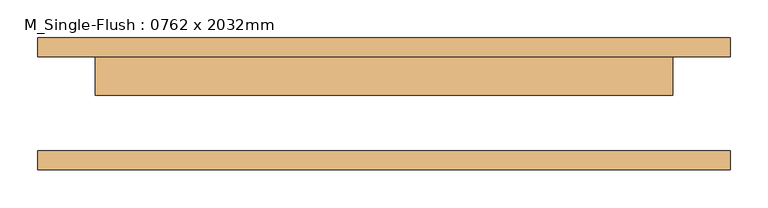
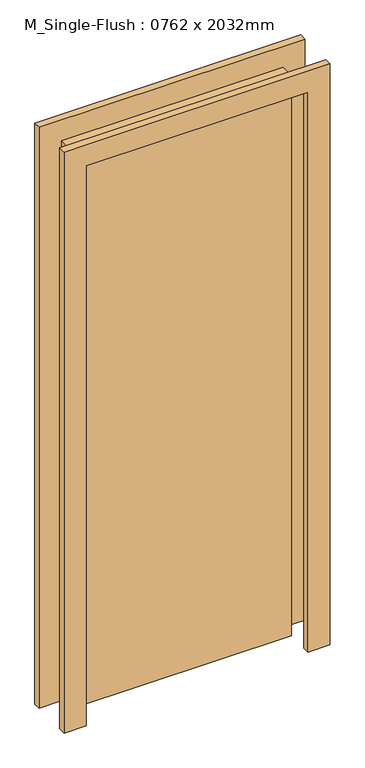
"""IFC4 building model written with IfcOpenShell, lengths in millimetres: door geometry, M_Single-Flush : 0762 x 2032mm."""

import ifcopenshell
import ifcopenshell.guid

model = None  # the IFC model being written
_history = None  # IfcOwnerHistory: only IFC2X3 demands one
_inside = {}  # id of a spatial element -> (the spatial element, [elements in it])
_under = {}  # id of a project, library or spatial element -> (it, [spatial elements below it])
_declared = {}  # id of a project -> (the project, [libraries it declares])
_typed = {}  # id of a type object -> (the type object, [elements of that type])
_made_of = {}  # id of a material, layer set ... -> (it, [elements and type objects made of it])


def new_model(schema):
    """Start an empty IFC model of exactly this schema.

    Asked for "IFC4X3", IfcOpenShell would pick the latest addendum, in which some entities
    have other attributes; the version numbers below select the first issue.
    IFC2X3 requires an IfcOwnerHistory on every rooted entity: one is made here for all.
    """
    global model, _history
    if schema == "IFC4X3":
        model = ifcopenshell.file(schema_version=(4, 3, 0, 0))
    else:
        model = ifcopenshell.file(schema=schema)
    _inside.clear()
    _under.clear()
    _declared.clear()
    _typed.clear()
    _made_of.clear()
    _history = None
    if model.schema == "IFC2X3":
        org = make("IfcOrganization", Name="unknown")
        user = make(
            "IfcPersonAndOrganization",
            ThePerson=make("IfcPerson", FamilyName="unknown"),
            TheOrganization=org,
        )
        app = make(
            "IfcApplication",
            ApplicationDeveloper=org,
            Version="unknown",
            ApplicationFullName="unknown",
            ApplicationIdentifier="unknown",
        )
        _history = make(
            "IfcOwnerHistory",
            OwningUser=user,
            OwningApplication=app,
            ChangeAction="ADDED",
            CreationDate=0,
        )
    return model


def make(cls, **values):
    """One entity of the class cls with the attributes given. An attribute that is None is left unset."""
    return model.create_entity(
        cls, **{name: value for name, value in values.items() if value is not None}
    )


def rooted(cls, **values):
    """An entity with a GlobalId (a new one), such as an element, a storey or a relation."""
    return make(cls, GlobalId=ifcopenshell.guid.new(), OwnerHistory=_history, **values)


def si_unit(unit_type, name, prefix=None):
    """IfcSIUnit, for example si_unit("LENGTHUNIT", "METRE", prefix="MILLI")."""
    return make("IfcSIUnit", UnitType=unit_type, Prefix=prefix, Name=name)


def assignment(units):
    """IfcUnitAssignment: the units of a project."""
    return None if units is None else make("IfcUnitAssignment", Units=units)


def point(xyz):
    """IfcCartesianPoint."""
    return None if xyz is None else make("IfcCartesianPoint", Coordinates=xyz)


def direction(xyz):
    """IfcDirection."""
    return None if xyz is None else make("IfcDirection", DirectionRatios=xyz)


def frame(location, z_axis=None, x_axis=None):
    """IfcAxis2Placement3D, a coordinate frame: its origin and axes. An axis left out is left unset."""
    return make(
        "IfcAxis2Placement3D",
        Location=point(location),
        Axis=direction(z_axis),
        RefDirection=direction(x_axis),
    )


def origin():
    """The frame at (0, 0, 0) with its axes left unset."""
    return frame((0.0, 0.0, 0.0))


def origin_with_axes():
    """The frame at (0, 0, 0) with the z axis (0, 0, 1) and the x axis (1, 0, 0) written out."""
    return frame((0.0, 0.0, 0.0), z_axis=(0.0, 0.0, 1.0), x_axis=(1.0, 0.0, 0.0))


def place(relative_to, where):
    """IfcLocalPlacement: puts the frame where relative to a parent placement (None: the world)."""
    return make(
        "IfcLocalPlacement", PlacementRelTo=relative_to, RelativePlacement=where
    )


def context(
    kind, dimensions, precision=None, world=None, true_north=None, identifier=None
):
    """IfcGeometricRepresentationContext, for example the 3D "Model" context."""
    return make(
        "IfcGeometricRepresentationContext",
        ContextIdentifier=identifier,
        ContextType=kind,
        CoordinateSpaceDimension=dimensions,
        Precision=precision,
        WorldCoordinateSystem=world,
        TrueNorth=true_north,
    )


def project(units=None, contexts=None):
    """IfcProject with its units and contexts."""
    return rooted(
        "IfcProject",
        Name="project",
        RepresentationContexts=contexts,
        UnitsInContext=assignment(units),
    )


def spatial(cls, under=None, at=None, **own):
    """A site, building, storey or space (cls), placed at a placement, below another one or the project."""
    s = rooted(cls, ObjectPlacement=at, **own)
    if under is not None:
        _under.setdefault(under.id(), (under, []))[1].append(s)
    return s


def polyline(points):
    """IfcPolyline through the points."""
    return make("IfcPolyline", Points=[point(p) for p in points])


def outline(outer, holes=None, kind="AREA"):
    """IfcArbitraryClosedProfileDef: a profile drawn as a closed curve; with holes, ...WithVoids."""
    if holes is None:
        return make("IfcArbitraryClosedProfileDef", ProfileType=kind, OuterCurve=outer)
    return make(
        "IfcArbitraryProfileDefWithVoids",
        ProfileType=kind,
        OuterCurve=outer,
        InnerCurves=holes,
    )


def extrude(swept, where, along, depth):
    """IfcExtrudedAreaSolid: the profile swept, set in the frame where, extruded along a direction by depth."""
    return make(
        "IfcExtrudedAreaSolid",
        SweptArea=swept,
        Position=where,
        ExtrudedDirection=direction(along),
        Depth=depth,
    )


def shape(context_of_items, identifier, shape_type, items):
    """IfcShapeRepresentation: the items that make up one representation, for example the "Body"."""
    return make(
        "IfcShapeRepresentation",
        ContextOfItems=context_of_items,
        RepresentationIdentifier=identifier,
        RepresentationType=shape_type,
        Items=items,
    )


def source(mapping_origin, context_of_items, identifier, shape_type, items):
    """IfcRepresentationMap: a shape defined once, which mapped items show again and again."""
    return make(
        "IfcRepresentationMap",
        MappingOrigin=mapping_origin,
        MappedRepresentation=shape(context_of_items, identifier, shape_type, items),
    )


def transform(
    local_origin,
    x_axis=None,
    y_axis=None,
    z_axis=None,
    scale=None,
    scale2=None,
    scale3=None,
    uniform=True,
):
    """IfcCartesianTransformationOperator3D, or its non-uniform kind. x_axis, y_axis, z_axis: its Axis1, 2, 3."""
    if uniform:
        return make(
            "IfcCartesianTransformationOperator3D",
            Axis1=direction(x_axis),
            Axis2=direction(y_axis),
            LocalOrigin=point(local_origin),
            Scale=scale,
            Axis3=direction(z_axis),
        )
    return make(
        "IfcCartesianTransformationOperator3DnonUniform",
        Axis1=direction(x_axis),
        Axis2=direction(y_axis),
        LocalOrigin=point(local_origin),
        Scale=scale,
        Axis3=direction(z_axis),
        Scale2=scale2,
        Scale3=scale3,
    )


def mapped(mapping_source, mapping_target):
    """IfcMappedItem: shows the shape of a source again, moved by a transform."""
    return make(
        "IfcMappedItem", MappingSource=mapping_source, MappingTarget=mapping_target
    )


def made_of(thing, what):
    """Note that an element or type object is made of a material, layer set ...; save() writes the relation."""
    if what is not None:
        _made_of.setdefault(what.id(), (what, []))[1].append(thing)
    return thing


def element(
    cls,
    number,
    at=None,
    inside=None,
    cuts=None,
    type_object=None,
    material=None,
    context=None,
    identifier="Body",
    shape_type=None,
    held_by="IfcProductDefinitionShape",
    body=None,
    shapes=None,
    **own,
):
    """One element of the class cls, such as IfcWall. Its Tag is "e" and its number.

    at: its placement. inside: the storey or other place that contains it. cuts: it is an
    opening in that element (IfcRelVoidsElement). A single representation is given by context,
    identifier, shape_type and body (its items); several are given by shapes. held_by: the class
    of the entity that holds the representations. save() writes the other relations.
    """
    e = rooted(cls, Tag="e%d" % number, ObjectPlacement=at, **own)
    if body is not None:
        shapes = [shape(context, identifier, shape_type, body)]
    if shapes is not None:
        e.Representation = make(held_by, Representations=shapes)
    if inside is not None:
        _inside.setdefault(inside.id(), (inside, []))[1].append(e)
    if cuts is not None:
        rooted(
            "IfcRelVoidsElement", RelatingBuildingElement=cuts, RelatedOpeningElement=e
        )
    if type_object is not None:
        _typed.setdefault(type_object.id(), (type_object, []))[1].append(e)
    return made_of(e, material)


def aggregate(whole, parts):
    """IfcRelAggregates: a whole, such as a stair, and the parts it consists of."""
    return rooted("IfcRelAggregates", RelatingObject=whole, RelatedObjects=parts)


def save(model, path):
    """Write the relations noted so far, then the file.

    IfcRelAggregates (storeys below a building ...), IfcRelContainedInSpatialStructure (elements
    in a storey), IfcRelDefinesByType, IfcRelAssociatesMaterial and IfcRelDeclares: one each for
    every whole, place, type object, material and project.
    """
    for whole, parts in _under.values():
        aggregate(whole, parts)
    for where, things in _inside.values():
        rooted(
            "IfcRelContainedInSpatialStructure",
            RelatedElements=things,
            RelatingStructure=where,
        )
    for kind, things in _typed.values():
        rooted("IfcRelDefinesByType", RelatedObjects=things, RelatingType=kind)
    for what, things in _made_of.values():
        rooted("IfcRelAssociatesMaterial", RelatedObjects=things, RelatingMaterial=what)
    for by, libraries in _declared.values():
        rooted("IfcRelDeclares", RelatingContext=by, RelatedDefinitions=libraries)
    model.write(path)


def m_single_flush_0762_x_2032mm_e53dc8c7(model_context):
    return source(origin(), model_context, "Body", "SweptSolid", [
        extrude(outline(polyline([(2108.0, -457.0), (0.0, -457.0), (0.0, -381.0), (2032.0, -381.0), (2032.0, 381.0), (0.0, 381.0), (0.0, 457.0), (2108.0, 457.0), (2108.0, -457.0)])), frame((0.0, 62.0, 0.0), z_axis=(0.0, 1.0, 0.0), x_axis=(0.0, 0.0, 1.0)), (0.0, 0.0, 1.0), 25.0),
        extrude(outline(polyline([(2108.0, 457.0), (2108.0, -457.0), (0.0, -457.0), (0.0, -381.0), (2032.0, -381.0), (2032.0, 381.0), (0.0, 381.0), (0.0, 457.0), (2108.0, 457.0)])), frame((0.0, -87.0, 0.0), z_axis=(0.0, 1.0, 0.0), x_axis=(0.0, 0.0, 1.0)), (0.0, 0.0, 1.0), 25.0),
        extrude(outline(polyline([(381.0, 11.0), (-381.0, 11.0), (-381.0, 62.0), (381.0, 62.0), (381.0, 11.0)])), origin_with_axes(), (0.0, 0.0, 1.0), 2032.0),
    ])


if __name__ == "__main__":
    model = new_model("IFC4")
    model_context = context("Model", 3, world=origin())
    ifc_project = project(units=[si_unit("LENGTHUNIT", "METRE", prefix="MILLI")], contexts=[model_context])
    site = spatial("IfcSite", under=ifc_project)
    building = spatial("IfcBuilding", under=site)
    placement = place(None, origin())
    m_single_flush_0762_x_2032mm_shape = m_single_flush_0762_x_2032mm_e53dc8c7(model_context)
    element("IfcDoor", 1, ObjectType="M_Single-Flush : 0762 x 2032mm", at=placement, inside=building, context=model_context, shape_type="MappedRepresentation", body=[
        mapped(m_single_flush_0762_x_2032mm_shape, transform((0.0, 0.0, 0.0), x_axis=(1.0, 0.0, 0.0), y_axis=(0.0, 1.0, 0.0), z_axis=(0.0, 0.0, 1.0))),
    ])
    save(model, "model.ifc")

# Revit data of these elements
# Type "M_Single-Flush : 0762 x 2032mm"
#   Manufacturer = "Manufacturer"
#   Type Mark = "28"
#   Construction Type = "Construction Type"
#   Fire Rating = "Fire Rating"
#   AccessibilityPerformance = "AccessibilityPerformance"
#   CodePerformance = "CodePerformance"
#   IsFireExit = "IsFireExit"
#   ConstructionType = "ConstructionType"
#   GlazingAreaFraction = "GlazingAreaFraction"
#   OperationType = "OperationType"
#   Area = "Area"
#   Color = "Color"
#   Constituents = "Constituents"
#   Features = "Features"
#   Finish = "Finish"
#   Grade = "Grade"
#   Material = "Material"
#   ModelReference = "ModelReference"
#   NominalHeight = "NominalHeight"
#   NominalLength = "NominalLength"
#   NominalWidth = "NominalWidth"
#   ProductionYear = "ProductionYear"
#   Reference = "Reference"
#   Shape = "Shape"
#   Size = "Size"
#   SustainabilityPerformance = "SustainabilityPerformance"
#   WarrantyDescription = "WarrantyDescription"
#   WarrantyDurationLabor = "WarrantyDurationLabor"
#   WarrantyDurationParts = "WarrantyDurationParts"
#   WarrantyGuarantorLabor = "WarrantyGuarantorLabor"
#   WarrantyGuarantorParts = "WarrantyGuarantorParts"
#   ExpectedLife = "ExpectedLife"
#   ReplacementCost = "ReplacementCost"
#   AssetAccountingType = "FIXED"
#   ModelLabel = "ModelLabel"
#   Thickness = 0.051 m
#   Height = 2.032 m
#   Trim Projection Ext = 0.025 m
#   Trim Projection Int = 0.025 m
#   Trim Width = 0.076 m
#   Width = 0.762 m
#   Door Material = Door - Panel
#   Frame Material = Door - Frame
#   Function = (empty or 0)
#   Wall Closure = (empty or 0)
# Element 1 (IfcDoor, "M_Single-Flush : 0762 x 2032mm")
#   Materials on its faces: "Door - Frame", "Door - Panel"
# Materials
#   "Door - Panel": class "Wood", colour RGB 210 159 95, transparency 0
#   "Door - Frame": class "Miscellaneous", colour RGB 118 70 51, transparency 0
